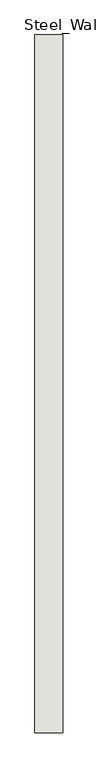
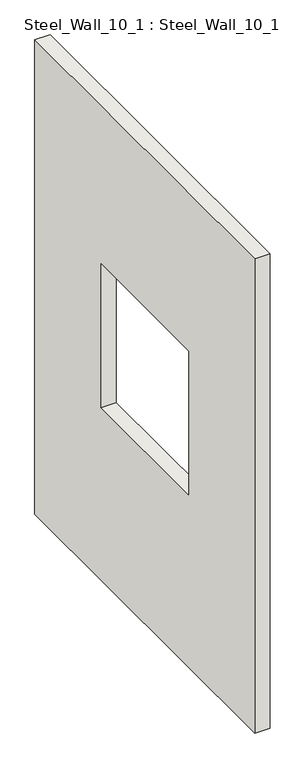
"""IFC4 building model written with IfcOpenShell, lengths in millimetres: wall geometry, Steel_Wall_10_1 : Steel_Wall_10_1."""

from ifc_helpers import new_model, si_unit, frame, origin, place, context, project, spatial, polyline, outline, extrude, source, transform, mapped, element, save


def steel_wall_10_1_steel_wall_10_1_b84ba1d7(model_context):
    return source(origin(), model_context, "Body", "SweptSolid", [
        extrude(outline(polyline([(9595.0, 3550.0), (12105.0, 3550.0), (12105.0, 250.0), (9595.0, 250.0), (9595.0, 3550.0)]), holes=[polyline([(11350.0, 2450.0), (10350.0, 2450.0), (10350.0, 1450.0), (11350.0, 1450.0), (11350.0, 2450.0)])]), frame((4265.0, 0.0, 0.0), z_axis=(1.0, 0.0, 0.0), x_axis=(0.0, 1.0, 0.0)), (0.0, 0.0, 1.0), 100.0),
    ])


if __name__ == "__main__":
    model = new_model("IFC4")
    model_context = context("Model", 3, world=origin())
    ifc_project = project(units=[si_unit("LENGTHUNIT", "METRE", prefix="MILLI")], contexts=[model_context])
    site = spatial("IfcSite", under=ifc_project)
    building = spatial("IfcBuilding", under=site)
    placement = place(None, origin())
    steel_wall_10_1_steel_wall_10_1_shape = steel_wall_10_1_steel_wall_10_1_b84ba1d7(model_context)
    element("IfcWall", 1, ObjectType="Steel_Wall_10_1 : Steel_Wall_10_1", at=placement, inside=building, context=model_context, shape_type="MappedRepresentation", body=[
        mapped(steel_wall_10_1_steel_wall_10_1_shape, transform((0.0, 0.0, 0.0), x_axis=(1.0, 0.0, 0.0), y_axis=(0.0, 1.0, 0.0), z_axis=(0.0, 0.0, 1.0))),
    ])
    save(model, "model.ifc")

# Revit data of these elements
# Type "Steel_Wall_10_1 : Steel_Wall_10_1"
#   NameOverride = "Steel_Wall_10_1"
# Element 1 (IfcWall, "Steel_Wall_10_1 : Steel_Wall_10_1")
#   Materials on its faces: "IfcSurfaceStyle #33"
# Materials
#   "IfcSurfaceStyle #33": class "Unassigned", colour RGB 214 214 214, transparency 0
